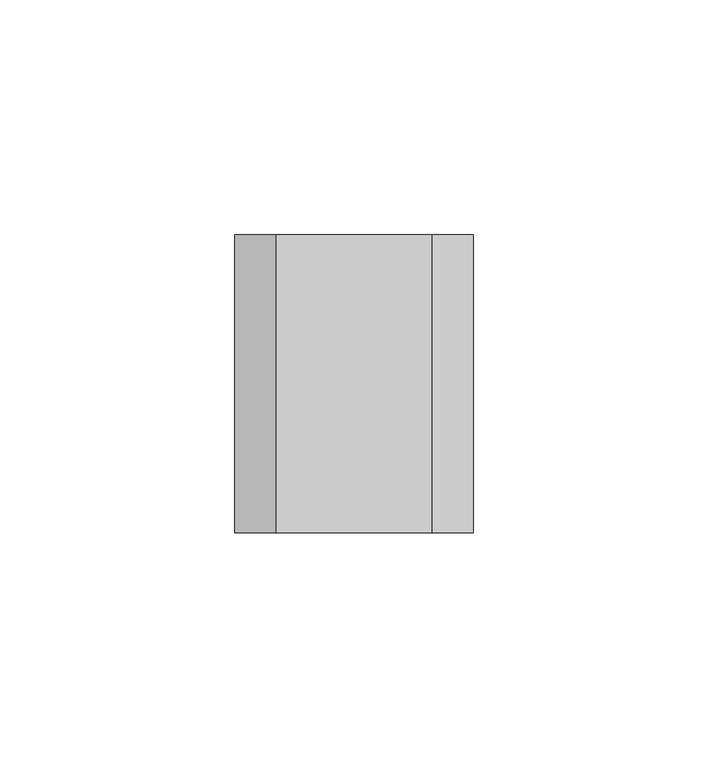
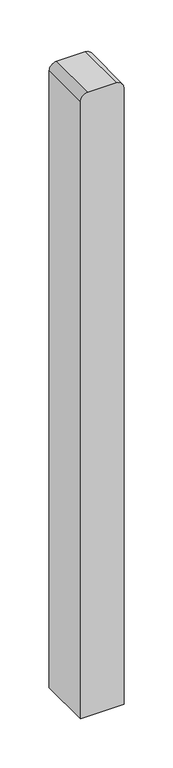
"""IFC4 building model written with IfcOpenShell, lengths in millimetres: proxy geometry, Generic Models 219:Generic Models 219:154155 : Generic Models 219:Generic Models 219:154155."""

from ifc_helpers import new_model, si_unit, point, frame, frame_2d, origin, place, context, project, spatial, polyline, circle_curve, trimmed, segment, composite_curve, outline, extrude, source, transform, mapped, element, save


def generic_models_a3779884(model_context):
    return source(origin(), model_context, "Body", "SweptSolid", [
        extrude(outline(composite_curve([segment(trimmed(circle_curve(frame_2d((2938.0611172, 7796.992413)), 8.8392), [point((2946.9003172, 7796.992413))], [point((2938.0611172, 7788.153213))], False, "CARTESIAN"), True, "CONTINUOUS"), segment(polyline([(2938.0611172, 7788.153213), (2175.4786907, 7788.153213), (2175.4786907, 7838.953213), (2938.0611172, 7838.953213)]), True, "CONTINUOUS"), segment(trimmed(circle_curve(frame_2d((2938.0611172, 7830.114013)), 8.8392), [point((2938.0611172, 7838.953213))], [point((2946.9003172, 7830.114013))], False, "CARTESIAN"), True, "CONTINUOUS"), segment(polyline([(2946.9003172, 7830.114013), (2946.9003172, 7796.992413)]), True, "CONTINUOUS")], self_intersect=False)), frame((0.0, 4691.511949, 0.0), z_axis=(0.0, 1.0, 0.0), x_axis=(0.0, 0.0, 1.0)), (0.0, 0.0, 1.0), 63.500874),
    ])


if __name__ == "__main__":
    model = new_model("IFC4")
    model_context = context("Model", 3, world=origin())
    ifc_project = project(units=[si_unit("LENGTHUNIT", "METRE", prefix="MILLI")], contexts=[model_context])
    site = spatial("IfcSite", under=ifc_project)
    building = spatial("IfcBuilding", under=site)
    placement = place(None, origin())
    generic_models_shape = generic_models_a3779884(model_context)
    element("IfcBuildingElementProxy", 1, Name="Generic Models 219:Generic Models 219:154155 : Generic Models 219:Generic Models 219:154155", ObjectType="Generic Models 219:Generic Models 219:154155 : Generic Models 219:Generic Models 219:154155", at=placement, inside=building, context=model_context, shape_type="MappedRepresentation", body=[
        mapped(generic_models_shape, transform((0.0, 0.0, 0.0), x_axis=(1.0, 0.0, 0.0), y_axis=(0.0, 1.0, 0.0), z_axis=(0.0, 0.0, 1.0))),
    ])
    save(model, "model.ifc")

# Revit data of these elements
# Type "Generic Models 219:Generic Models 219:154155 : Generic Models 219:Generic Models 219:154155"
#   NameOverride = "Generic Models 219:Generic Models 219:154155"
#   ObjectTypeOverride = "Generic Models 219:Generic Models 219"
#   Reference = "Generic Models 219"
#   Category = "Generic Models"
#   Tag = "154155"
# Element 1 (IfcBuildingElementProxy, "Generic Models 219:Generic Models 219:154155 : Generic Models 219:Generic Models 219:154155")
#   Materials on its faces: "_2x3 STEEL PROFILE - METALIZED, PRIMED & PAINTED (COLOR PER ARCHITECT)"
# Materials
#   "_2x3 STEEL PROFILE - METALIZED, PRIMED & PAINTED (COLOR PER ARCHITECT)": class "Metal", colour RGB 199 199 199, transparency 0, Description = "Structural steel 50ksi", Cost = 0
